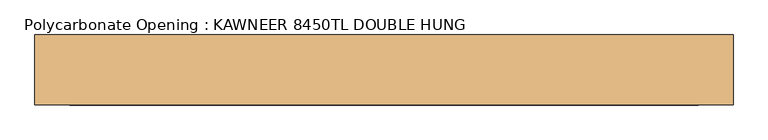
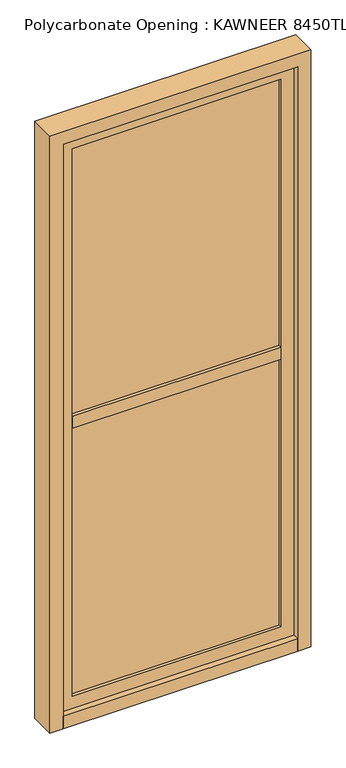
"""IFC4 building model written with IfcOpenShell, lengths in millimetres: door geometry, Polycarbonate Opening : KAWNEER 8450TL DOUBLE HUNG."""

import ifcopenshell
import ifcopenshell.guid

model = None  # the IFC model being written
_history = None  # IfcOwnerHistory: only IFC2X3 demands one
_inside = {}  # id of a spatial element -> (the spatial element, [elements in it])
_under = {}  # id of a project, library or spatial element -> (it, [spatial elements below it])
_declared = {}  # id of a project -> (the project, [libraries it declares])
_typed = {}  # id of a type object -> (the type object, [elements of that type])
_made_of = {}  # id of a material, layer set ... -> (it, [elements and type objects made of it])


def new_model(schema):
    """Start an empty IFC model of exactly this schema.

    Asked for "IFC4X3", IfcOpenShell would pick the latest addendum, in which some entities
    have other attributes; the version numbers below select the first issue.
    IFC2X3 requires an IfcOwnerHistory on every rooted entity: one is made here for all.
    """
    global model, _history
    if schema == "IFC4X3":
        model = ifcopenshell.file(schema_version=(4, 3, 0, 0))
    else:
        model = ifcopenshell.file(schema=schema)
    _inside.clear()
    _under.clear()
    _declared.clear()
    _typed.clear()
    _made_of.clear()
    _history = None
    if model.schema == "IFC2X3":
        org = make("IfcOrganization", Name="unknown")
        user = make(
            "IfcPersonAndOrganization",
            ThePerson=make("IfcPerson", FamilyName="unknown"),
            TheOrganization=org,
        )
        app = make(
            "IfcApplication",
            ApplicationDeveloper=org,
            Version="unknown",
            ApplicationFullName="unknown",
            ApplicationIdentifier="unknown",
        )
        _history = make(
            "IfcOwnerHistory",
            OwningUser=user,
            OwningApplication=app,
            ChangeAction="ADDED",
            CreationDate=0,
        )
    return model


def make(cls, **values):
    """One entity of the class cls with the attributes given. An attribute that is None is left unset."""
    return model.create_entity(
        cls, **{name: value for name, value in values.items() if value is not None}
    )


def rooted(cls, **values):
    """An entity with a GlobalId (a new one), such as an element, a storey or a relation."""
    return make(cls, GlobalId=ifcopenshell.guid.new(), OwnerHistory=_history, **values)


def si_unit(unit_type, name, prefix=None):
    """IfcSIUnit, for example si_unit("LENGTHUNIT", "METRE", prefix="MILLI")."""
    return make("IfcSIUnit", UnitType=unit_type, Prefix=prefix, Name=name)


def assignment(units):
    """IfcUnitAssignment: the units of a project."""
    return None if units is None else make("IfcUnitAssignment", Units=units)


def point(xyz):
    """IfcCartesianPoint."""
    return None if xyz is None else make("IfcCartesianPoint", Coordinates=xyz)


def direction(xyz):
    """IfcDirection."""
    return None if xyz is None else make("IfcDirection", DirectionRatios=xyz)


def frame(location, z_axis=None, x_axis=None):
    """IfcAxis2Placement3D, a coordinate frame: its origin and axes. An axis left out is left unset."""
    return make(
        "IfcAxis2Placement3D",
        Location=point(location),
        Axis=direction(z_axis),
        RefDirection=direction(x_axis),
    )


def origin():
    """The frame at (0, 0, 0) with its axes left unset."""
    return frame((0.0, 0.0, 0.0))


def origin_with_axes():
    """The frame at (0, 0, 0) with the z axis (0, 0, 1) and the x axis (1, 0, 0) written out."""
    return frame((0.0, 0.0, 0.0), z_axis=(0.0, 0.0, 1.0), x_axis=(1.0, 0.0, 0.0))


def place(relative_to, where):
    """IfcLocalPlacement: puts the frame where relative to a parent placement (None: the world)."""
    return make(
        "IfcLocalPlacement", PlacementRelTo=relative_to, RelativePlacement=where
    )


def context(
    kind, dimensions, precision=None, world=None, true_north=None, identifier=None
):
    """IfcGeometricRepresentationContext, for example the 3D "Model" context."""
    return make(
        "IfcGeometricRepresentationContext",
        ContextIdentifier=identifier,
        ContextType=kind,
        CoordinateSpaceDimension=dimensions,
        Precision=precision,
        WorldCoordinateSystem=world,
        TrueNorth=true_north,
    )


def project(units=None, contexts=None):
    """IfcProject with its units and contexts."""
    return rooted(
        "IfcProject",
        Name="project",
        RepresentationContexts=contexts,
        UnitsInContext=assignment(units),
    )


def spatial(cls, under=None, at=None, **own):
    """A site, building, storey or space (cls), placed at a placement, below another one or the project."""
    s = rooted(cls, ObjectPlacement=at, **own)
    if under is not None:
        _under.setdefault(under.id(), (under, []))[1].append(s)
    return s


def polyline(points):
    """IfcPolyline through the points."""
    return make("IfcPolyline", Points=[point(p) for p in points])


def outline(outer, holes=None, kind="AREA"):
    """IfcArbitraryClosedProfileDef: a profile drawn as a closed curve; with holes, ...WithVoids."""
    if holes is None:
        return make("IfcArbitraryClosedProfileDef", ProfileType=kind, OuterCurve=outer)
    return make(
        "IfcArbitraryProfileDefWithVoids",
        ProfileType=kind,
        OuterCurve=outer,
        InnerCurves=holes,
    )


def extrude(swept, where, along, depth):
    """IfcExtrudedAreaSolid: the profile swept, set in the frame where, extruded along a direction by depth."""
    return make(
        "IfcExtrudedAreaSolid",
        SweptArea=swept,
        Position=where,
        ExtrudedDirection=direction(along),
        Depth=depth,
    )


def shape(context_of_items, identifier, shape_type, items):
    """IfcShapeRepresentation: the items that make up one representation, for example the "Body"."""
    return make(
        "IfcShapeRepresentation",
        ContextOfItems=context_of_items,
        RepresentationIdentifier=identifier,
        RepresentationType=shape_type,
        Items=items,
    )


def source(mapping_origin, context_of_items, identifier, shape_type, items):
    """IfcRepresentationMap: a shape defined once, which mapped items show again and again."""
    return make(
        "IfcRepresentationMap",
        MappingOrigin=mapping_origin,
        MappedRepresentation=shape(context_of_items, identifier, shape_type, items),
    )


def transform(
    local_origin,
    x_axis=None,
    y_axis=None,
    z_axis=None,
    scale=None,
    scale2=None,
    scale3=None,
    uniform=True,
):
    """IfcCartesianTransformationOperator3D, or its non-uniform kind. x_axis, y_axis, z_axis: its Axis1, 2, 3."""
    if uniform:
        return make(
            "IfcCartesianTransformationOperator3D",
            Axis1=direction(x_axis),
            Axis2=direction(y_axis),
            LocalOrigin=point(local_origin),
            Scale=scale,
            Axis3=direction(z_axis),
        )
    return make(
        "IfcCartesianTransformationOperator3DnonUniform",
        Axis1=direction(x_axis),
        Axis2=direction(y_axis),
        LocalOrigin=point(local_origin),
        Scale=scale,
        Axis3=direction(z_axis),
        Scale2=scale2,
        Scale3=scale3,
    )


def mapped(mapping_source, mapping_target):
    """IfcMappedItem: shows the shape of a source again, moved by a transform."""
    return make(
        "IfcMappedItem", MappingSource=mapping_source, MappingTarget=mapping_target
    )


def made_of(thing, what):
    """Note that an element or type object is made of a material, layer set ...; save() writes the relation."""
    if what is not None:
        _made_of.setdefault(what.id(), (what, []))[1].append(thing)
    return thing


def element(
    cls,
    number,
    at=None,
    inside=None,
    cuts=None,
    type_object=None,
    material=None,
    context=None,
    identifier="Body",
    shape_type=None,
    held_by="IfcProductDefinitionShape",
    body=None,
    shapes=None,
    **own,
):
    """One element of the class cls, such as IfcWall. Its Tag is "e" and its number.

    at: its placement. inside: the storey or other place that contains it. cuts: it is an
    opening in that element (IfcRelVoidsElement). A single representation is given by context,
    identifier, shape_type and body (its items); several are given by shapes. held_by: the class
    of the entity that holds the representations. save() writes the other relations.
    """
    e = rooted(cls, Tag="e%d" % number, ObjectPlacement=at, **own)
    if body is not None:
        shapes = [shape(context, identifier, shape_type, body)]
    if shapes is not None:
        e.Representation = make(held_by, Representations=shapes)
    if inside is not None:
        _inside.setdefault(inside.id(), (inside, []))[1].append(e)
    if cuts is not None:
        rooted(
            "IfcRelVoidsElement", RelatingBuildingElement=cuts, RelatedOpeningElement=e
        )
    if type_object is not None:
        _typed.setdefault(type_object.id(), (type_object, []))[1].append(e)
    return made_of(e, material)


def aggregate(whole, parts):
    """IfcRelAggregates: a whole, such as a stair, and the parts it consists of."""
    return rooted("IfcRelAggregates", RelatingObject=whole, RelatedObjects=parts)


def save(model, path):
    """Write the relations noted so far, then the file.

    IfcRelAggregates (storeys below a building ...), IfcRelContainedInSpatialStructure (elements
    in a storey), IfcRelDefinesByType, IfcRelAssociatesMaterial and IfcRelDeclares: one each for
    every whole, place, type object, material and project.
    """
    for whole, parts in _under.values():
        aggregate(whole, parts)
    for where, things in _inside.values():
        rooted(
            "IfcRelContainedInSpatialStructure",
            RelatedElements=things,
            RelatingStructure=where,
        )
    for kind, things in _typed.values():
        rooted("IfcRelDefinesByType", RelatedObjects=things, RelatingType=kind)
    for what, things in _made_of.values():
        rooted("IfcRelAssociatesMaterial", RelatedObjects=things, RelatingMaterial=what)
    for by, libraries in _declared.values():
        rooted("IfcRelDeclares", RelatingContext=by, RelatedDefinitions=libraries)
    model.write(path)


def polycarbonate_opening_kawneer_8450tl_double_hung_daf3f652(model_context):
    return source(origin(), model_context, "Body", "SweptSolid", [
        extrude(outline(polyline([(457.2, 12.7), (457.2, -12.7), (-457.2, -12.7), (-457.2, 12.7), (457.2, 12.7)])), frame((0.0, 0.0, 50.8), z_axis=(0.0, 0.0, 1.0), x_axis=(1.0, 0.0, 0.0)), (0.0, 0.0, 1.0), 2356.0492241),
        extrude(outline(polyline([(2406.8492241, -457.2), (0.0, -457.2), (0.0, 457.2), (2406.8492241, 457.2), (2406.8492241, -457.2)]), holes=[polyline([(101.6, 406.4), (101.6, -406.4), (2356.0492241, -406.4), (2356.0492241, 406.4), (101.6, 406.4)])]), frame((0.0, -25.4, 0.0), z_axis=(0.0, 1.0, 0.0), x_axis=(0.0, 0.0, 1.0)), (0.0, 0.0, 1.0), 50.8),
        extrude(outline(polyline([(2457.6492241, 508.0), (2457.6492241, -508.0), (0.0, -508.0), (0.0, -457.2), (2406.8492241, -457.2), (2406.8492241, 457.2), (0.0, 457.2), (0.0, 508.0), (2457.6492241, 508.0)])), frame((0.0, -50.8, 0.0), z_axis=(0.0, 1.0, 0.0), x_axis=(0.0, 0.0, 1.0)), (0.0, 0.0, 1.0), 101.6),
        extrude(outline(polyline([(457.2, 50.8), (457.2, -50.8), (-457.2, -50.8), (-457.2, 50.8), (457.2, 50.8)])), origin_with_axes(), (0.0, 0.0, 1.0), 50.8),
        extrude(outline(polyline([(406.4, 25.4), (406.4, -25.4), (-406.4, -25.4), (-406.4, 25.4), (406.4, 25.4)])), frame((0.0, 0.0, 1203.424612), z_axis=(0.0, 0.0, 1.0), x_axis=(1.0, 0.0, 0.0)), (0.0, 0.0, 1.0), 50.8),
    ])


if __name__ == "__main__":
    model = new_model("IFC4")
    model_context = context("Model", 3, world=origin())
    ifc_project = project(units=[si_unit("LENGTHUNIT", "METRE", prefix="MILLI")], contexts=[model_context])
    site = spatial("IfcSite", under=ifc_project)
    building = spatial("IfcBuilding", under=site)
    placement = place(None, origin())
    polycarbonate_opening_kawneer_8450tl_double_hung_shape = polycarbonate_opening_kawneer_8450tl_double_hung_daf3f652(model_context)
    element("IfcDoor", 1, ObjectType="Polycarbonate Opening : KAWNEER 8450TL DOUBLE HUNG", at=placement, inside=building, context=model_context, shape_type="MappedRepresentation", body=[
        mapped(polycarbonate_opening_kawneer_8450tl_double_hung_shape, transform((0.0, 0.0, 0.0), x_axis=(1.0, 0.0, 0.0), y_axis=(0.0, 1.0, 0.0), z_axis=(0.0, 0.0, 1.0))),
    ])
    save(model, "model.ifc")

# Revit data of these elements
# Type "Polycarbonate Opening : KAWNEER 8450TL DOUBLE HUNG"
#   Type Mark = "59"
#   OD_DS_Door_Material = "ALUM./GLAZING"
#   OD_DS_Door_Type = "STOREFRONT - DOUBLE HUNG WINDOW"
#   OD_DS_Lockset = "POLE OPERATOR HARDWARE FOR TOP SASH; BOTTOM SASH MECHANICALLY FIXED"
#   Analytic Construction = "<None>"
#   offset [instance default] = 0' - 2"
#   Stile = 0' - 2"
#   Mullion Width = 0' - 2"
#   Mullion Depth = 0' - 4"
#   Opening Size [instance default] = 5' - 1.50212"
#   Door Width [instance default] = 5' - 1.50212"
#   Window ON/OFF = no
#   Door On/Off = yes
#   Mullion Material = DOUBLE HUNG (CLEAR ANODIZED ALUM) - TEMPERED INSULATED GLAZING (CARDINAL GLASS LoĒ²-240\nOR EQUIVALENT)
#   Glass Material = TEMPERED INSULATED GLAZING (CARDINAL GLASS LoĒ²-240\nOR EQUIVALENT)
#   Door Material = DOUBLE HUNG (CLEAR ANODIZED ALUM) - TEMPERED INSULATED GLAZING (CARDINAL GLASS LoĒ²-240\nOR EQUIVALENT)
# Element 1 (IfcDoor, "Polycarbonate Opening : KAWNEER 8450TL DOUBLE HUNG")
#   offset = 0' - 0"
#   Materials on its faces: "DOUBLE HUNG (CLEAR ANODIZED ALUM) - TEMPERED INSULATED GLAZING (CARDINAL GLASS LoĒ²-240\nOR EQUIVALENT)", "TEMPERED INSULATED GLAZING (CARDINAL GLASS LoĒ²-240\nOR EQUIVALENT)"
# Materials
#   "DOUBLE HUNG (CLEAR ANODIZED ALUM) - TEMPERED INSULATED GLAZING (CARDINAL GLASS LoĒ²-240\nOR EQUIVALENT)": class "Metal", colour RGB 244 244 244, transparency 0, Description = "Aluminum 6061", Cost = 0
#   "TEMPERED INSULATED GLAZING (CARDINAL GLASS LoĒ²-240\nOR EQUIVALENT)": class "Glass", colour RGB 196 205 210, transparency 0.85, Description = "Soda Lime Glass", Cost = 0
